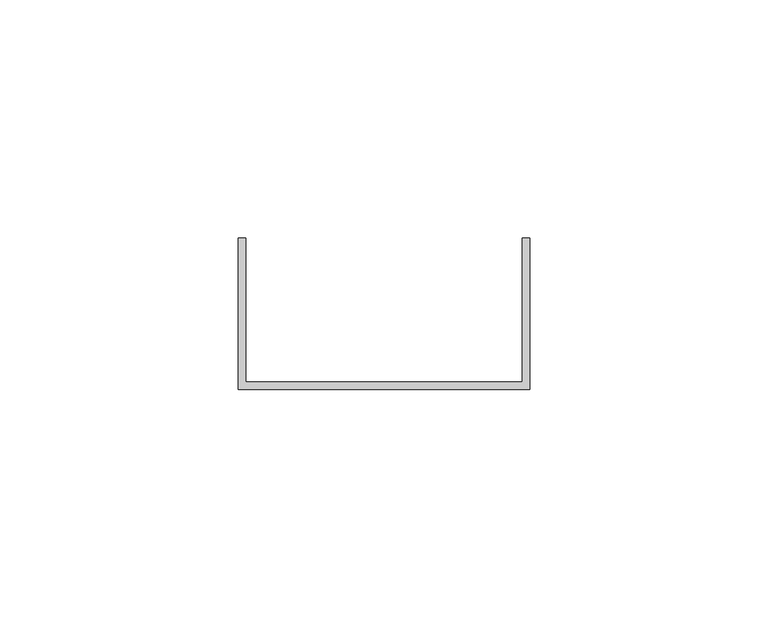
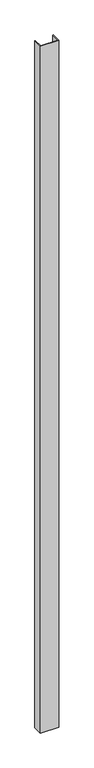
"""IFC4 building model written with IfcOpenShell, lengths in millimetres: proxy geometry, Generic Models 7:Generic Models 1:3:Generic Models 1:3 : Generic Models 7:Generic Models 1:305549:3:Generic Models 1:3:Generic Models 1:3 : Generic Models 7:Generic Models 1:305549:3 : Generic Models 7:Generic Models 1:3:Generic Models 1:3 : Generic Models 7:Generic Models 1:305549:301244:47 : Generic Models 7:Generic Models 1:3:Generic Models 1:3 : Generic Models 7:Generic Models 1:305549:3:Generic Models 1:3:Generic Models 1:3 : Generic Models 7:Generic Models 1:305549:3 : Generic Models 7:Generic Models 1:3:Generic Models 1:3 : Generic Models 7:Generic Models 1:305549:301244:308848."""

from ifc_helpers import new_model, si_unit, frame, origin, place, context, project, spatial, polyline, outline, extrude, source, transform, mapped, element, save


def generic_models_d51cfe46(model_context):
    return source(origin(), model_context, "Body", "SweptSolid", [
        extrude(outline(polyline([(560350.5804739, -579013.3913841), (560289.4617239, -579013.3913841), (560289.4617239, -578981.6413841), (560291.0492239, -578981.6413841), (560291.0492239, -579011.8038841), (560348.9929739, -579011.8038841), (560348.9929739, -578981.6413841), (560350.5804739, -578981.6413841), (560350.5804739, -579013.3913841)])), frame((0.0, 0.0, 3721.1), z_axis=(0.0, 0.0, 1.0), x_axis=(1.0, 0.0, 0.0)), (0.0, 0.0, 1.0), 2430.9324376),
    ])


if __name__ == "__main__":
    model = new_model("IFC4")
    model_context = context("Model", 3, world=origin())
    ifc_project = project(units=[si_unit("LENGTHUNIT", "METRE", prefix="MILLI")], contexts=[model_context])
    site = spatial("IfcSite", under=ifc_project)
    building = spatial("IfcBuilding", under=site)
    placement = place(None, origin())
    generic_models_shape = generic_models_d51cfe46(model_context)
    element("IfcBuildingElementProxy", 1, Name="Generic Models 7:Generic Models 1:3:Generic Models 1:3 : Generic Models 7:Generic Models 1:305549:3:Generic Models 1:3:Generic Models 1:3 : Generic Models 7:Generic Models 1:305549:3 : Generic Models 7:Generic Models 1:3:Generic Models 1:3 : Generic Models 7:Generic Models 1:305549:301244:47 : Generic Models 7:Generic Models 1:3:Generic Models 1:3 : Generic Models 7:Generic Models 1:305549:3:Generic Models 1:3:Generic Models 1:3 : Generic Models 7:Generic Models 1:305549:3 : Generic Models 7:Generic Models 1:3:Generic Models 1:3 : Generic Models 7:Generic Models 1:305549:301244:308848", ObjectType="Generic Models 7:Generic Models 1:3:Generic Models 1:3 : Generic Models 7:Generic Models 1:305549:3:Generic Models 1:3:Generic Models 1:3 : Generic Models 7:Generic Models 1:305549:3 : Generic Models 7:Generic Models 1:3:Generic Models 1:3 : Generic Models 7:Generic Models 1:305549:301244:47 : Generic Models 7:Generic Models 1:3:Generic Models 1:3 : Generic Models 7:Generic Models 1:305549:3:Generic Models 1:3:Generic Models 1:3 : Generic Models 7:Generic Models 1:305549:3 : Generic Models 7:Generic Models 1:3:Generic Models 1:3 : Generic Models 7:Generic Models 1:305549:301244:308848", at=placement, inside=building, context=model_context, shape_type="MappedRepresentation", body=[
        mapped(generic_models_shape, transform((0.0, 0.0, 0.0), x_axis=(1.0, 0.0, 0.0), y_axis=(0.0, 1.0, 0.0), z_axis=(0.0, 0.0, 1.0))),
    ])
    save(model, "model.ifc")

# Revit data of these elements
# Type "Generic Models 7:Generic Models 1:3:Generic Models 1:3 : Generic Models 7:Generic Models 1:305549:3:Generic Models 1:3:Generic Models 1:3 : Generic Models 7:Generic Models 1:305549:3 : Generic Models 7:Generic Models 1:3:Generic Models 1:3 : Generic Models 7:Generic Models 1:305549:301244:47 : Generic Models 7:Generic Models 1:3:Generic Models 1:3 : Generic Models 7:Generic Models 1:305549:3:Generic Models 1:3:Generic Models 1:3 : Generic Models 7:Generic Models 1:305549:3 : Generic Models 7:Generic Models 1:3:Generic Models 1:3 : Generic Models 7:Generic Models 1:305549:301244:308848"
#   NameOverride = "Generic Models 7:Generic Models 1:3:Generic Models 1:3 : Generic Models 7:Generic Models 1:305549:3:Generic Models 1:3:Generic Models 1:3 : Generic Models 7:Generic Models 1:305549:3 : Generic Models 7:Generic Models 1:3:Generic Models 1:3 : Generic Models 7:Generic Models 1:305549:301244:308848"
#   ObjectTypeOverride = "Generic Models 1:3:Generic Models 1:3 : Generic Models 7:Generic Models 1:305549:3 : Generic Models 7:Generic Models 1:3:Generic Models 1:3 : Generic Models 7:Generic Models 1:305549:301244"
#   Reference = "Generic Models 1"
#   Tag = "308848"
# Element 1 (IfcBuildingElementProxy, "Generic Models 7:Generic Models 1:3:Generic Models 1:3 : Generic Models 7:Generic Models 1:305549:3:Generic Models 1:3:Generic Models 1:3 : Generic Models 7:Generic Models 1:305549:3 : Generic Models 7:Generic Models 1:3:Generic Models 1:3 : Generic Models 7:Generic Models 1:305549:301244:47 : Generic Models 7:Generic Models 1:3:Generic Models 1:3 : Generic Models 7:Generic Models 1:305549:3:Generic Models 1:3:Generic Models 1:3 : Generic Models 7:Generic Models 1:305549:3 : Generic Models 7:Generic Models 1:3:Generic Models 1:3 : Generic Models 7:Generic Models 1:305549:301244:308848")
#   Materials on its faces: "GALVANIZED U-CHANNEL (250T125-33)"
# Materials
#   "GALVANIZED U-CHANNEL (250T125-33)": class "Unassigned", colour RGB 202 201 200, transparency 0, Keynote = "M05451300.02", Cost = 0
